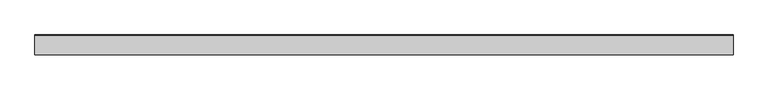
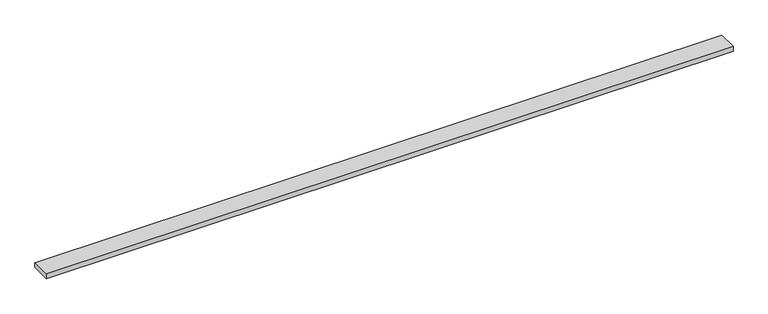
"""IFC4 building model written with IfcOpenShell, lengths in millimetres: proxy geometry, Generic Models 7:Generic Models 1:2:Generic Models 1:2 : Generic Models 7:Generic Models 1:337419:2 : Generic Models 7:Generic Models 1:2:Generic Models 1:2 : Generic Models 7:Generic Models 1:337419:306751."""

from ifc_helpers import new_model, si_unit, frame, origin, place, context, project, spatial, polyline, outline, extrude, source, transform, mapped, element, save


def generic_models_7d058cf7(model_context):
    return source(origin(), model_context, "Body", "SweptSolid", [
        extrude(outline(polyline([(-578740.3413841, 3693.8479167), (-578740.3413841, 3731.9479167), (-578603.2165864, 3731.9479167), (-578600.6413841, 3729.3727144), (-578600.6413841, 3693.8479167), (-578740.3413841, 3693.8479167)])), frame((591306.0367239, 0.0, 0.0), z_axis=(1.0, 0.0, 0.0), x_axis=(0.0, 1.0, 0.0)), (0.0, 0.0, 1.0), 4876.8),
    ])


if __name__ == "__main__":
    model = new_model("IFC4")
    model_context = context("Model", 3, world=origin())
    ifc_project = project(units=[si_unit("LENGTHUNIT", "METRE", prefix="MILLI")], contexts=[model_context])
    site = spatial("IfcSite", under=ifc_project)
    building = spatial("IfcBuilding", under=site)
    placement = place(None, origin())
    generic_models_shape = generic_models_7d058cf7(model_context)
    element("IfcBuildingElementProxy", 1, Name="Generic Models 7:Generic Models 1:2:Generic Models 1:2 : Generic Models 7:Generic Models 1:337419:2 : Generic Models 7:Generic Models 1:2:Generic Models 1:2 : Generic Models 7:Generic Models 1:337419:306751", ObjectType="Generic Models 7:Generic Models 1:2:Generic Models 1:2 : Generic Models 7:Generic Models 1:337419:2 : Generic Models 7:Generic Models 1:2:Generic Models 1:2 : Generic Models 7:Generic Models 1:337419:306751", at=placement, inside=building, context=model_context, shape_type="MappedRepresentation", body=[
        mapped(generic_models_shape, transform((0.0, 0.0, 0.0), x_axis=(1.0, 0.0, 0.0), y_axis=(0.0, 1.0, 0.0), z_axis=(0.0, 0.0, 1.0))),
    ])
    save(model, "model.ifc")

# Revit data of these elements
# Type "Generic Models 7:Generic Models 1:2:Generic Models 1:2 : Generic Models 7:Generic Models 1:337419:2 : Generic Models 7:Generic Models 1:2:Generic Models 1:2 : Generic Models 7:Generic Models 1:337419:306751"
#   NameOverride = "Generic Models 7:Generic Models 1:2:Generic Models 1:2 : Generic Models 7:Generic Models 1:337419:306751"
#   ObjectTypeOverride = "Generic Models 1:2 : Generic Models 7:Generic Models 1:337419"
#   Reference = "Generic Models 1"
#   Tag = "306751"
# Element 1 (IfcBuildingElementProxy, "Generic Models 7:Generic Models 1:2:Generic Models 1:2 : Generic Models 7:Generic Models 1:337419:2 : Generic Models 7:Generic Models 1:2:Generic Models 1:2 : Generic Models 7:Generic Models 1:337419:306751")
#   Materials on its faces: "FIRE RETARDTANT WOOD BLOCKING - SIZE AS NECESSARY"
# Materials
#   "FIRE RETARDTANT WOOD BLOCKING - SIZE AS NECESSARY": class "Wood", colour RGB 144 113 62, transparency 0, Description = "Pinus Echinata", Cost = 0
